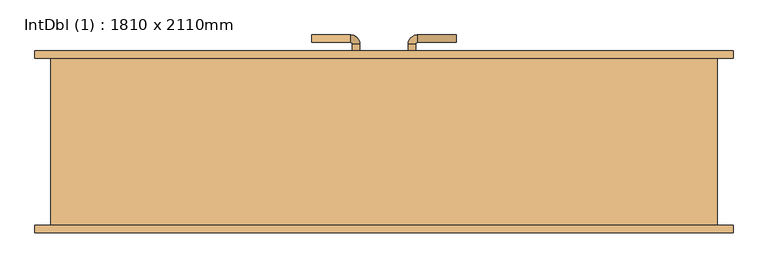
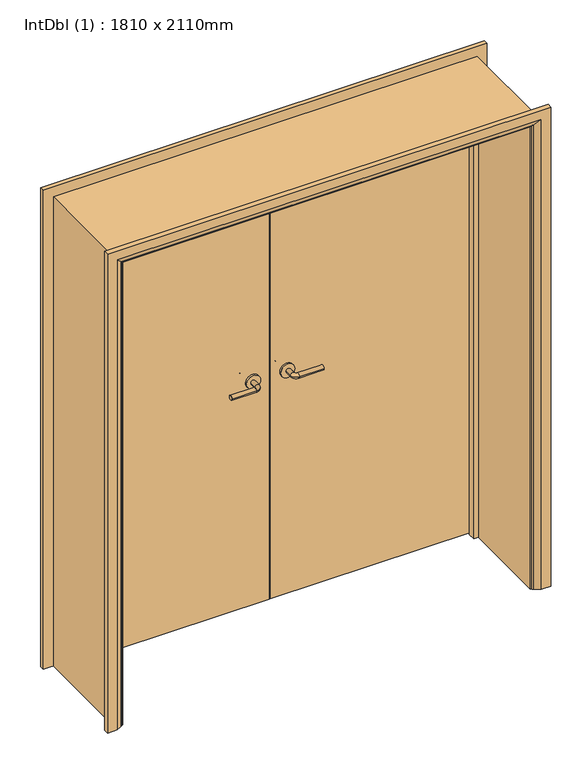
"""IFC4 building model written with IfcOpenShell, lengths in millimetres: door geometry, IntDbl (1) : 1810 x 2110mm."""

from ifc_helpers import new_model, si_unit, point, frame, frame_2d, origin, place, context, project, spatial, polyline, circle_curve, ellipse_curve, trimmed, segment, composite_curve, outline, extrude, faceted_brep, source, transform, mapped, element, save
from ifc_brep_helpers import plane_surface, cylinder_surface, revolved_surface, advanced_brep


def intdbl_1_1810_x_2110mm_24fdf151(model_context):
    return source(origin(), model_context, "Body", "SolidModel", [
        advanced_brep(
        [(-65.0, 185.0, 1007.0), (-85.0, 185.0, 1007.0), (-65.0, 155.0, 1007.0), (-85.0, 155.0, 1007.0), (-90.0, 150.0, 1007.0), (-90.0, 130.0, 1007.0), (-195.0, 130.0, 1007.0), (-195.0, 150.0, 1007.0)],
        [
            (0, 1, circle_curve(frame((-75.0, 185.0, 1007.0), z_axis=(0.0, 1.0, 0.0), x_axis=(-1.0, 0.0, 0.0)), 10.0)),
            (1, 0, circle_curve(frame((-75.0, 185.0, 1007.0), z_axis=(0.0, 1.0, 0.0), x_axis=(-1.0, 0.0, 0.0)), 10.0)),
            (0, 2),
            (2, 3, circle_curve(frame((-75.0, 155.0, 1007.0), z_axis=(0.0, 1.0, 0.0), x_axis=(-1.0, 0.0, 0.0)), 10.0)),
            (3, 1),
            (3, 2, circle_curve(frame((-75.0, 155.0, 1007.0), z_axis=(0.0, 1.0, 0.0), x_axis=(-1.0, 0.0, 0.0)), 10.0)),
            (4, 3, circle_curve(frame((-90.0, 155.0, 1007.0), z_axis=(0.0, 0.0, 1.0), x_axis=(1.0, 0.0, 0.0)), 5.0)),
            (2, 5, circle_curve(frame((-90.0, 155.0, 1007.0), z_axis=(0.0, 0.0, -1.0), x_axis=(1.0, 0.0, 0.0)), 25.0)),
            (5, 4, circle_curve(frame((-90.0, 140.0, 1007.0), z_axis=(1.0, 0.0, 0.0), x_axis=(0.0, 1.0, 0.0)), 10.0)),
            (4, 5, circle_curve(frame((-90.0, 140.0, 1007.0), z_axis=(1.0, 0.0, 0.0), x_axis=(0.0, 1.0, 0.0)), 10.0)),
            (6, 7, circle_curve(frame((-195.0, 140.0, 1007.0), z_axis=(-1.0, 0.0, 0.0), x_axis=(0.0, 1.0, 0.0)), 10.0)),
            (7, 6, circle_curve(frame((-195.0, 140.0, 1007.0), z_axis=(-1.0, 0.0, 0.0), x_axis=(0.0, 1.0, 0.0)), 10.0)),
            (5, 6),
            (7, 4),
        ],
        [
            plane_surface(frame((-75.0, 185.0, 1007.0), z_axis=(0.0, 1.0, 0.0), x_axis=(0.0, 0.0, 1.0))),
            cylinder_surface(frame((-75.0, 185.0, 1007.0), z_axis=(0.0, 1.0, 0.0), x_axis=(-1.0, 0.0, 0.0)), 10.0),
            revolved_surface(trimmed(ellipse_curve(frame((-75.0, 155.0, 1007.0), z_axis=(0.0, 1.0, 0.0), x_axis=(-1.0, 0.0, 0.0)), 10.0, 10.0), [point((-65.0, 155.0, 1007.0))], [point((-85.0, 155.0, 1007.0))], True, "CARTESIAN"), (-90.0, 155.0, 1007.0), (0.0, 0.0, -1.0)),
            revolved_surface(trimmed(ellipse_curve(frame((-75.0, 155.0, 1007.0), z_axis=(0.0, 1.0, 0.0), x_axis=(-1.0, 0.0, 0.0)), 10.0, 10.0), [point((-85.0, 155.0, 1007.0))], [point((-65.0, 155.0, 1007.0))], True, "CARTESIAN"), (-90.0, 155.0, 1007.0), (0.0, 0.0, -1.0)),
            plane_surface(frame((-195.0, 140.0, 1007.0), z_axis=(-1.0, 0.0, 0.0), x_axis=(0.0, 0.0, 1.0))),
            cylinder_surface(frame((-90.0, 140.0, 1007.0), z_axis=(1.0, 0.0, 0.0), x_axis=(0.0, 1.0, 0.0)), 10.0),
        ],
        [
            (0, [[1, 2]]),
            (1, [[-1, 3, 4, 5]]),
            (1, [[-2, -5, 6, -3]]),
            (2, [[7, -4, 8, 9]]),
            (3, [[-8, -6, -7, 10]]),
            (4, [[11, 12]]),
            (5, [[-9, 13, -12, 14]]),
            (5, [[-10, -14, -11, -13]]),
        ],
    ),
        extrude(outline(composite_curve([segment(trimmed(circle_curve(frame_2d((1007.0, -72.5)), 30.0), [point((1007.0, -42.5))], [point((1007.0, -102.5))], False, "CARTESIAN"), True, "CONTINUOUS"), segment(trimmed(circle_curve(frame_2d((1007.0, -72.5)), 30.0), [point((1007.0, -102.5))], [point((1007.0, -42.5))], False, "CARTESIAN"), True, "CONTINUOUS")], self_intersect=False)), frame((0.0, 185.0, 0.0), z_axis=(0.0, 1.0, 0.0), x_axis=(0.0, 0.0, 1.0)), (0.0, 0.0, 1.0), 8.0),
        advanced_brep(
        [(-65.0, 233.0, 1007.0), (-85.0, 233.0, 1007.0), (-85.0, 263.0, 1007.0), (-65.0, 263.0, 1007.0), (-90.0, 268.0, 1007.0), (-90.0, 288.0, 1007.0), (-195.0, 288.0, 1007.0), (-195.0, 268.0, 1007.0)],
        [
            (0, 1, circle_curve(frame((-75.0, 233.0, 1007.0), z_axis=(0.0, -1.0, 0.0), x_axis=(-1.0, 0.0, 0.0)), 10.0)),
            (1, 0, circle_curve(frame((-75.0, 233.0, 1007.0), z_axis=(0.0, -1.0, 0.0), x_axis=(-1.0, 0.0, 0.0)), 10.0)),
            (1, 2),
            (2, 3, circle_curve(frame((-75.0, 263.0, 1007.0), z_axis=(0.0, -1.0, 0.0), x_axis=(-1.0, 0.0, 0.0)), 10.0)),
            (3, 0),
            (3, 2, circle_curve(frame((-75.0, 263.0, 1007.0), z_axis=(0.0, -1.0, 0.0), x_axis=(-1.0, 0.0, 0.0)), 10.0)),
            (4, 5, circle_curve(frame((-90.0, 278.0, 1007.0), z_axis=(1.0, 0.0, 0.0), x_axis=(0.0, -1.0, 0.0)), 10.0)),
            (5, 3, circle_curve(frame((-90.0, 263.0, 1007.0), z_axis=(0.0, 0.0, -1.0), x_axis=(1.0, 0.0, 0.0)), 25.0)),
            (2, 4, circle_curve(frame((-90.0, 263.0, 1007.0), z_axis=(0.0, 0.0, 1.0), x_axis=(1.0, 0.0, 0.0)), 5.0)),
            (5, 4, circle_curve(frame((-90.0, 278.0, 1007.0), z_axis=(1.0, 0.0, 0.0), x_axis=(0.0, -1.0, 0.0)), 10.0)),
            (6, 7, circle_curve(frame((-195.0, 278.0, 1007.0), z_axis=(-1.0, 0.0, 0.0), x_axis=(0.0, -1.0, 0.0)), 10.0)),
            (7, 6, circle_curve(frame((-195.0, 278.0, 1007.0), z_axis=(-1.0, 0.0, 0.0), x_axis=(0.0, -1.0, 0.0)), 10.0)),
            (4, 7),
            (6, 5),
        ],
        [
            plane_surface(frame((-75.0, 233.0, 1007.0), z_axis=(0.0, -1.0, 0.0), x_axis=(0.0, 0.0, 1.0))),
            cylinder_surface(frame((-75.0, 233.0, 1007.0), z_axis=(0.0, -1.0, 0.0), x_axis=(-1.0, 0.0, 0.0)), 10.0),
            revolved_surface(trimmed(ellipse_curve(frame((-75.0, 263.0, 1007.0), z_axis=(0.0, 1.0, 0.0), x_axis=(-1.0, 0.0, 0.0)), 10.0, 10.0), [point((-65.0, 263.0, 1007.0))], [point((-85.0, 263.0, 1007.0))], True, "CARTESIAN"), (-90.0, 263.0, 1007.0), (0.0, 0.0, -1.0)),
            revolved_surface(trimmed(ellipse_curve(frame((-75.0, 263.0, 1007.0), z_axis=(0.0, 1.0, 0.0), x_axis=(-1.0, 0.0, 0.0)), 10.0, 10.0), [point((-85.0, 263.0, 1007.0))], [point((-65.0, 263.0, 1007.0))], True, "CARTESIAN"), (-90.0, 263.0, 1007.0), (0.0, 0.0, -1.0)),
            plane_surface(frame((-195.0, 278.0, 1007.0), z_axis=(-1.0, 0.0, 0.0), x_axis=(0.0, 0.0, 1.0))),
            cylinder_surface(frame((-90.0, 278.0, 1007.0), z_axis=(1.0, 0.0, 0.0), x_axis=(0.0, -1.0, 0.0)), 10.0),
        ],
        [
            (0, [[1, 2]]),
            (1, [[3, 4, 5, -2]]),
            (1, [[-5, 6, -3, -1]]),
            (2, [[7, 8, -4, 9]]),
            (3, [[10, -9, -6, -8]]),
            (4, [[11, 12]]),
            (5, [[13, -11, 14, -7]]),
            (5, [[-14, -12, -13, -10]]),
        ],
    ),
        extrude(outline(composite_curve([segment(trimmed(circle_curve(frame_2d((1007.0, -72.5)), 30.0), [point((1007.0, -42.5))], [point((1007.0, -102.5))], False, "CARTESIAN"), True, "CONTINUOUS"), segment(trimmed(circle_curve(frame_2d((1007.0, -72.5)), 30.0), [point((1007.0, -102.5))], [point((1007.0, -42.5))], False, "CARTESIAN"), True, "CONTINUOUS")], self_intersect=False)), frame((0.0, 225.0, 0.0), z_axis=(0.0, 1.0, 0.0), x_axis=(0.0, 0.0, 1.0)), (0.0, 0.0, 1.0), 8.0),
        advanced_brep(
        [(65.0, 185.0, 1007.0), (85.0, 185.0, 1007.0), (85.0, 155.0, 1007.0), (65.0, 155.0, 1007.0), (90.0, 150.0, 1007.0), (90.0, 130.0, 1007.0), (195.0, 130.0, 1007.0), (195.0, 150.0, 1007.0)],
        [
            (0, 1, circle_curve(frame((75.0, 185.0, 1007.0), z_axis=(0.0, 1.0, 0.0), x_axis=(1.0, 0.0, 0.0)), 10.0)),
            (1, 0, circle_curve(frame((75.0, 185.0, 1007.0), z_axis=(0.0, 1.0, 0.0), x_axis=(1.0, 0.0, 0.0)), 10.0)),
            (1, 2),
            (2, 3, circle_curve(frame((75.0, 155.0, 1007.0), z_axis=(0.0, 1.0, 0.0), x_axis=(1.0, 0.0, 0.0)), 10.0)),
            (3, 0),
            (3, 2, circle_curve(frame((75.0, 155.0, 1007.0), z_axis=(0.0, 1.0, 0.0), x_axis=(1.0, 0.0, 0.0)), 10.0)),
            (4, 5, circle_curve(frame((90.0, 140.0, 1007.0), z_axis=(-1.0, 0.0, 0.0), x_axis=(0.0, 1.0, 0.0)), 10.0)),
            (5, 3, circle_curve(frame((90.0, 155.0, 1007.0), z_axis=(0.0, 0.0, -1.0), x_axis=(-1.0, 0.0, 0.0)), 25.0)),
            (2, 4, circle_curve(frame((90.0, 155.0, 1007.0), z_axis=(0.0, 0.0, 1.0), x_axis=(-1.0, 0.0, 0.0)), 5.0)),
            (5, 4, circle_curve(frame((90.0, 140.0, 1007.0), z_axis=(-1.0, 0.0, 0.0), x_axis=(0.0, 1.0, 0.0)), 10.0)),
            (6, 7, circle_curve(frame((195.0, 140.0, 1007.0), z_axis=(1.0, 0.0, 0.0), x_axis=(0.0, 1.0, 0.0)), 10.0)),
            (7, 6, circle_curve(frame((195.0, 140.0, 1007.0), z_axis=(1.0, 0.0, 0.0), x_axis=(0.0, 1.0, 0.0)), 10.0)),
            (4, 7),
            (6, 5),
        ],
        [
            plane_surface(frame((75.0, 185.0, 1007.0), z_axis=(0.0, 1.0, 0.0), x_axis=(0.0, 0.0, 1.0))),
            cylinder_surface(frame((75.0, 185.0, 1007.0), z_axis=(0.0, 1.0, 0.0), x_axis=(1.0, 0.0, 0.0)), 10.0),
            revolved_surface(trimmed(ellipse_curve(frame((75.0, 155.0, 1007.0), z_axis=(0.0, -1.0, 0.0), x_axis=(1.0, 0.0, 0.0)), 10.0, 10.0), [point((65.0, 155.0, 1007.0))], [point((85.0, 155.0, 1007.0))], True, "CARTESIAN"), (90.0, 155.0, 1007.0), (0.0, 0.0, -1.0)),
            revolved_surface(trimmed(ellipse_curve(frame((75.0, 155.0, 1007.0), z_axis=(0.0, -1.0, 0.0), x_axis=(1.0, 0.0, 0.0)), 10.0, 10.0), [point((85.0, 155.0, 1007.0))], [point((65.0, 155.0, 1007.0))], True, "CARTESIAN"), (90.0, 155.0, 1007.0), (0.0, 0.0, -1.0)),
            plane_surface(frame((195.0, 140.0, 1007.0), z_axis=(1.0, 0.0, 0.0), x_axis=(0.0, 0.0, 1.0))),
            cylinder_surface(frame((90.0, 140.0, 1007.0), z_axis=(-1.0, 0.0, 0.0), x_axis=(0.0, 1.0, 0.0)), 10.0),
        ],
        [
            (0, [[1, 2]]),
            (1, [[3, 4, 5, -2]]),
            (1, [[-5, 6, -3, -1]]),
            (2, [[7, 8, -4, 9]]),
            (3, [[10, -9, -6, -8]]),
            (4, [[11, 12]]),
            (5, [[13, -11, 14, -7]]),
            (5, [[-14, -12, -13, -10]]),
        ],
    ),
        extrude(outline(composite_curve([segment(trimmed(circle_curve(frame_2d((1007.0, 72.5)), 30.0), [point((1007.0, 42.5))], [point((1007.0, 102.5))], False, "CARTESIAN"), True, "CONTINUOUS"), segment(trimmed(circle_curve(frame_2d((1007.0, 72.5)), 30.0), [point((1007.0, 102.5))], [point((1007.0, 42.5))], False, "CARTESIAN"), True, "CONTINUOUS")], self_intersect=False)), frame((0.0, 185.0, 0.0), z_axis=(0.0, 1.0, 0.0), x_axis=(0.0, 0.0, 1.0)), (0.0, 0.0, 1.0), 8.0),
        advanced_brep(
        [(65.0, 233.0, 1007.0), (85.0, 233.0, 1007.0), (65.0, 263.0, 1007.0), (85.0, 263.0, 1007.0), (90.0, 268.0, 1007.0), (90.0, 288.0, 1007.0), (195.0, 288.0, 1007.0), (195.0, 268.0, 1007.0)],
        [
            (0, 1, circle_curve(frame((75.0, 233.0, 1007.0), z_axis=(0.0, -1.0, 0.0), x_axis=(1.0, 0.0, 0.0)), 10.0)),
            (1, 0, circle_curve(frame((75.0, 233.0, 1007.0), z_axis=(0.0, -1.0, 0.0), x_axis=(1.0, 0.0, 0.0)), 10.0)),
            (0, 2),
            (2, 3, circle_curve(frame((75.0, 263.0, 1007.0), z_axis=(0.0, -1.0, 0.0), x_axis=(1.0, 0.0, 0.0)), 10.0)),
            (3, 1),
            (3, 2, circle_curve(frame((75.0, 263.0, 1007.0), z_axis=(0.0, -1.0, 0.0), x_axis=(1.0, 0.0, 0.0)), 10.0)),
            (4, 3, circle_curve(frame((90.0, 263.0, 1007.0), z_axis=(0.0, 0.0, 1.0), x_axis=(-1.0, 0.0, 0.0)), 5.0)),
            (2, 5, circle_curve(frame((90.0, 263.0, 1007.0), z_axis=(0.0, 0.0, -1.0), x_axis=(-1.0, 0.0, 0.0)), 25.0)),
            (5, 4, circle_curve(frame((90.0, 278.0, 1007.0), z_axis=(-1.0, 0.0, 0.0), x_axis=(0.0, -1.0, 0.0)), 10.0)),
            (4, 5, circle_curve(frame((90.0, 278.0, 1007.0), z_axis=(-1.0, 0.0, 0.0), x_axis=(0.0, -1.0, 0.0)), 10.0)),
            (6, 7, circle_curve(frame((195.0, 278.0, 1007.0), z_axis=(1.0, 0.0, 0.0), x_axis=(0.0, -1.0, 0.0)), 10.0)),
            (7, 6, circle_curve(frame((195.0, 278.0, 1007.0), z_axis=(1.0, 0.0, 0.0), x_axis=(0.0, -1.0, 0.0)), 10.0)),
            (5, 6),
            (7, 4),
        ],
        [
            plane_surface(frame((75.0, 233.0, 1007.0), z_axis=(0.0, -1.0, 0.0), x_axis=(0.0, 0.0, 1.0))),
            cylinder_surface(frame((75.0, 233.0, 1007.0), z_axis=(0.0, -1.0, 0.0), x_axis=(1.0, 0.0, 0.0)), 10.0),
            revolved_surface(trimmed(ellipse_curve(frame((75.0, 263.0, 1007.0), z_axis=(0.0, -1.0, 0.0), x_axis=(1.0, 0.0, 0.0)), 10.0, 10.0), [point((65.0, 263.0, 1007.0))], [point((85.0, 263.0, 1007.0))], True, "CARTESIAN"), (90.0, 263.0, 1007.0), (0.0, 0.0, -1.0)),
            revolved_surface(trimmed(ellipse_curve(frame((75.0, 263.0, 1007.0), z_axis=(0.0, -1.0, 0.0), x_axis=(1.0, 0.0, 0.0)), 10.0, 10.0), [point((85.0, 263.0, 1007.0))], [point((65.0, 263.0, 1007.0))], True, "CARTESIAN"), (90.0, 263.0, 1007.0), (0.0, 0.0, -1.0)),
            plane_surface(frame((195.0, 278.0, 1007.0), z_axis=(1.0, 0.0, 0.0), x_axis=(0.0, 0.0, 1.0))),
            cylinder_surface(frame((90.0, 278.0, 1007.0), z_axis=(-1.0, 0.0, 0.0), x_axis=(0.0, -1.0, 0.0)), 10.0),
        ],
        [
            (0, [[1, 2]]),
            (1, [[-1, 3, 4, 5]]),
            (1, [[-2, -5, 6, -3]]),
            (2, [[7, -4, 8, 9]]),
            (3, [[-8, -6, -7, 10]]),
            (4, [[11, 12]]),
            (5, [[-9, 13, -12, 14]]),
            (5, [[-10, -14, -11, -13]]),
        ],
    ),
        extrude(outline(composite_curve([segment(trimmed(circle_curve(frame_2d((1007.0, 72.5)), 30.0), [point((1007.0, 42.5))], [point((1007.0, 102.5))], False, "CARTESIAN"), True, "CONTINUOUS"), segment(trimmed(circle_curve(frame_2d((1007.0, 72.5)), 30.0), [point((1007.0, 102.5))], [point((1007.0, 42.5))], False, "CARTESIAN"), True, "CONTINUOUS")], self_intersect=False)), frame((0.0, 225.0, 0.0), z_axis=(0.0, 1.0, 0.0), x_axis=(0.0, 0.0, 1.0)), (0.0, 0.0, 1.0), 8.0),
        advanced_brep(
        [(-940.0, -245.0, 0.0), (-940.0, -225.0, 0.0), (-870.0, -225.0, 0.0), (-874.0, -231.0, 0.0), (-900.0, -245.0, 0.0), (-940.0, -245.0, 2145.0), (-940.0, -225.0, 2145.0), (940.0, -225.0, 2145.0), (940.0, -225.0, 0.0), (870.0, -225.0, 0.0), (870.0, -225.0, 2075.0), (-870.0, -225.0, 2075.0), (-874.0, -231.0, 2079.0), (-900.0, -245.0, 2105.0), (900.0, -245.0, 2105.0), (900.0, -245.0, 0.0), (940.0, -245.0, 0.0), (940.0, -245.0, 2145.0), (874.0, -231.0, 0.0), (874.0, -231.0, 2079.0)],
        [
            (0, 1),
            (1, 2),
            (2, 3, circle_curve(frame((-878.0, -224.0, 0.0), z_axis=(0.0, 0.0, -1.0), x_axis=(-1.0, 0.0, 0.0)), 8.0622577)),
            (3, 4),
            (4, 0),
            (0, 5),
            (5, 6),
            (6, 1),
            (6, 7),
            (7, 8),
            (8, 9),
            (9, 10),
            (10, 11),
            (11, 2),
            (11, 12, ellipse_curve(frame((-878.0, -224.0, 2083.0), z_axis=(-0.7071067811865475, 0.0, -0.7071067811865475), x_axis=(0.7071067811865474, 0.0, -0.7071067811865476)), 11.4017543, 8.0622577)),
            (12, 3),
            (12, 13),
            (13, 4),
            (13, 14),
            (14, 15),
            (15, 16),
            (16, 17),
            (17, 5),
            (7, 17),
            (16, 8),
            (15, 18),
            (18, 9, circle_curve(frame((878.0, -224.0, 0.0), z_axis=(0.0, 0.0, -1.0), x_axis=(1.0, 0.0, 0.0)), 8.0622577)),
            (19, 10, ellipse_curve(frame((878.0, -224.0, 2083.0), z_axis=(0.7071067811865475, 0.0, -0.7071067811865475), x_axis=(0.7071067811865474, 0.0, 0.7071067811865476)), 11.4017543, 8.0622577)),
            (18, 19),
            (14, 19),
            (19, 12),
        ],
        [
            plane_surface(frame((-870.0, -225.0, 0.0), z_axis=(0.0, 0.0, -1.0), x_axis=(0.0, -1.0, 0.0))),
            plane_surface(frame((-940.0, -245.0, 0.0), z_axis=(-1.0, 0.0, 0.0), x_axis=(0.0, 0.0, 1.0))),
            plane_surface(frame((-940.0, -225.0, 0.0), z_axis=(0.0, 1.0, 0.0), x_axis=(0.0, 0.0, 1.0))),
            cylinder_surface(frame((-878.0, -224.0, 0.0), z_axis=(0.0, 0.0, -1.0), x_axis=(-1.0, 0.0, 0.0)), 8.0622577),
            plane_surface(frame((-874.0, -231.0, 0.0), z_axis=(0.4740998230350183, -0.8804710999221749, 0.0), x_axis=(0.0, 0.0, 1.0))),
            plane_surface(frame((-900.0, -245.0, 0.0), z_axis=(0.0, -1.0, 0.0), x_axis=(0.0, 0.0, 1.0))),
            plane_surface(frame((940.0, -245.0, 2145.0), z_axis=(1.0, 0.0, 0.0), x_axis=(0.0, 0.0, -1.0))),
            plane_surface(frame((870.0, -225.0, 0.0), z_axis=(0.0, 0.0, -1.0), x_axis=(0.0, -1.0, 0.0))),
            cylinder_surface(frame((878.0, -224.0, 2075.0), z_axis=(0.0, 0.0, 1.0), x_axis=(1.0, 0.0, 0.0)), 8.0622577),
            plane_surface(frame((874.0, -231.0, 2079.0), z_axis=(-0.4740998230350183, -0.8804710999221749, 0.0), x_axis=(0.0, 0.0, -1.0))),
            plane_surface(frame((-940.0, -245.0, 2145.0), z_axis=(0.0, 0.0, 1.0), x_axis=(1.0, 0.0, 0.0))),
            cylinder_surface(frame((-870.0, -224.0, 2083.0), z_axis=(-1.0, 0.0, 0.0), x_axis=(0.0, 0.0, 1.0)), 8.0622577),
            plane_surface(frame((-874.0, -231.0, 2079.0), z_axis=(0.0, -0.8804710999221749, -0.4740998230350183), x_axis=(1.0, 0.0, 0.0))),
        ],
        [
            (0, [[1, 2, 3, 4, 5]]),
            (1, [[-1, 6, 7, 8]]),
            (2, [[-2, -8, 9, 10, 11, 12, 13, 14]]),
            (3, [[-3, -14, 15, 16]]),
            (4, [[-4, -16, 17, 18]]),
            (5, [[-5, -18, 19, 20, 21, 22, 23, -6]]),
            (6, [[24, -22, 25, -10]]),
            (7, [[-21, 26, 27, -11, -25]]),
            (8, [[28, -12, -27, 29]]),
            (9, [[30, -29, -26, -20]]),
            (10, [[-7, -23, -24, -9]]),
            (11, [[-15, -13, -28, 31]]),
            (12, [[-17, -31, -30, -19]]),
        ],
    ),
        advanced_brep(
        [(940.0, 245.0, 0.0), (940.0, 225.0, 0.0), (870.0, 225.0, 0.0), (874.0, 231.0, 0.0), (900.0, 245.0, 0.0), (940.0, 245.0, 2145.0), (940.0, 225.0, 2145.0), (-940.0, 225.0, 2145.0), (-940.0, 225.0, 0.0), (-870.0, 225.0, 0.0), (-870.0, 225.0, 2075.0), (870.0, 225.0, 2075.0), (874.0, 231.0, 2079.0), (900.0, 245.0, 2105.0), (-900.0, 245.0, 2105.0), (-900.0, 245.0, 0.0), (-940.0, 245.0, 0.0), (-940.0, 245.0, 2145.0), (-874.0, 231.0, 0.0), (-874.0, 231.0, 2079.0)],
        [
            (0, 1),
            (1, 2),
            (2, 3, circle_curve(frame((878.0, 224.0, 0.0), z_axis=(0.0, 0.0, -1.0), x_axis=(1.0, 0.0, 0.0)), 8.0622577)),
            (3, 4),
            (4, 0),
            (0, 5),
            (5, 6),
            (6, 1),
            (6, 7),
            (7, 8),
            (8, 9),
            (9, 10),
            (10, 11),
            (11, 2),
            (11, 12, ellipse_curve(frame((878.0, 224.0, 2083.0), z_axis=(0.7071067811865475, 0.0, -0.7071067811865475), x_axis=(-0.7071067811865474, 0.0, -0.7071067811865476)), 11.4017543, 8.0622577)),
            (12, 3),
            (12, 13),
            (13, 4),
            (13, 14),
            (14, 15),
            (15, 16),
            (16, 17),
            (17, 5),
            (7, 17),
            (16, 8),
            (15, 18),
            (18, 9, circle_curve(frame((-878.0, 224.0, 0.0), z_axis=(0.0, 0.0, -1.0), x_axis=(-1.0, 0.0, 0.0)), 8.0622577)),
            (19, 10, ellipse_curve(frame((-878.0, 224.0, 2083.0), z_axis=(-0.7071067811865475, 0.0, -0.7071067811865475), x_axis=(-0.7071067811865474, 0.0, 0.7071067811865476)), 11.4017543, 8.0622577)),
            (18, 19),
            (14, 19),
            (19, 12),
        ],
        [
            plane_surface(frame((870.0, 225.0, 0.0), z_axis=(0.0, 0.0, -1.0), x_axis=(0.0, -1.0, 0.0))),
            plane_surface(frame((940.0, 245.0, 0.0), z_axis=(1.0, 0.0, 0.0), x_axis=(0.0, 0.0, 1.0))),
            plane_surface(frame((940.0, 225.0, 0.0), z_axis=(0.0, -1.0, 0.0), x_axis=(0.0, 0.0, 1.0))),
            cylinder_surface(frame((878.0, 224.0, 0.0), z_axis=(0.0, 0.0, -1.0), x_axis=(1.0, 0.0, 0.0)), 8.0622577),
            plane_surface(frame((874.0, 231.0, 0.0), z_axis=(-0.4740998230350126, 0.8804710999221779, 0.0), x_axis=(0.0, 0.0, 1.0))),
            plane_surface(frame((900.0, 245.0, 0.0), z_axis=(0.0, 1.0, 0.0), x_axis=(0.0, 0.0, 1.0))),
            plane_surface(frame((-940.0, 245.0, 2145.0), z_axis=(-1.0, 0.0, 0.0), x_axis=(0.0, 0.0, -1.0))),
            plane_surface(frame((-870.0, 225.0, 0.0), z_axis=(0.0, 0.0, -1.0), x_axis=(0.0, -1.0, 0.0))),
            cylinder_surface(frame((-878.0, 224.0, 2075.0), z_axis=(0.0, 0.0, 1.0), x_axis=(-1.0, 0.0, 0.0)), 8.0622577),
            plane_surface(frame((-874.0, 231.0, 2079.0), z_axis=(0.4740998230350183, 0.8804710999221749, 0.0), x_axis=(0.0, 0.0, -1.0))),
            plane_surface(frame((940.0, 245.0, 2145.0), z_axis=(0.0, 0.0, 1.0), x_axis=(-1.0, 0.0, 0.0))),
            cylinder_surface(frame((870.0, 224.0, 2083.0), z_axis=(1.0, 0.0, 0.0), x_axis=(0.0, 0.0, 1.0)), 8.0622577),
            plane_surface(frame((874.0, 231.0, 2079.0), z_axis=(0.0, 0.8804710999221763, -0.4740998230350154), x_axis=(-1.0, 0.0, 0.0))),
        ],
        [
            (0, [[1, 2, 3, 4, 5]]),
            (1, [[-1, 6, 7, 8]]),
            (2, [[-2, -8, 9, 10, 11, 12, 13, 14]]),
            (3, [[-3, -14, 15, 16]]),
            (4, [[-4, -16, 17, 18]]),
            (5, [[-5, -18, 19, 20, 21, 22, 23, -6]]),
            (6, [[24, -22, 25, -10]]),
            (7, [[-21, 26, 27, -11, -25]]),
            (8, [[28, -12, -27, 29]]),
            (9, [[30, -29, -26, -20]]),
            (10, [[-7, -23, -24, -9]]),
            (11, [[-15, -13, -28, 31]]),
            (12, [[-17, -31, -30, -19]]),
        ],
    ),
        faceted_brep([(-846.0, 190.0, 0.0), (-846.0, 158.0, 0.0), (-865.0, 158.0, 0.0), (-865.0, 190.0, 0.0), (-846.0, 190.0, 2051.0), (-846.0, 158.0, 2051.0), (-865.0, 158.0, 2070.0), (-865.0, 190.0, 2070.0), (846.0, 190.0, 0.0), (865.0, 190.0, 0.0), (865.0, 158.0, 0.0), (846.0, 158.0, 0.0), (846.0, 190.0, 2051.0), (865.0, 190.0, 2070.0), (865.0, 158.0, 2070.0), (846.0, 158.0, 2051.0)], [[[0, 1, 2, 3]], [[1, 0, 4, 5]], [[2, 1, 5, 6]], [[3, 2, 6, 7]], [[0, 3, 7, 4]], [[8, 9, 10, 11]], [[12, 13, 9, 8]], [[13, 14, 10, 9]], [[14, 15, 11, 10]], [[15, 12, 8, 11]], [[5, 4, 12, 15]], [[6, 5, 15, 14]], [[7, 6, 14, 13]], [[4, 7, 13, 12]]]),
        extrude(outline(polyline([(2102.0, -897.0), (0.0, -897.0), (0.0, -865.0), (2070.0, -865.0), (2070.0, 865.0), (0.0, 865.0), (0.0, 897.0), (2102.0, 897.0), (2102.0, -897.0)])), frame((0.0, -225.0, 0.0), z_axis=(0.0, 1.0, 0.0), x_axis=(0.0, 0.0, 1.0)), (0.0, 0.0, 1.0), 450.0),
        extrude(outline(polyline([(-1.5, 193.0), (-862.0, 193.0), (-862.0, 225.0), (-1.5, 225.0), (-1.5, 193.0)])), frame((0.0, 0.0, 5.753223), z_axis=(0.0, 0.0, 1.0), x_axis=(1.0, 0.0, 0.0)), (0.0, 0.0, 1.0), 2061.246777),
        extrude(outline(polyline([(862.0, 193.0), (1.5, 193.0), (1.5, 225.0), (862.0, 225.0), (862.0, 193.0)])), frame((0.0, 0.0, 5.753223), z_axis=(0.0, 0.0, 1.0), x_axis=(1.0, 0.0, 0.0)), (0.0, 0.0, 1.0), 2061.246777),
    ])


if __name__ == "__main__":
    model = new_model("IFC4")
    model_context = context("Model", 3, world=origin())
    ifc_project = project(units=[si_unit("LENGTHUNIT", "METRE", prefix="MILLI")], contexts=[model_context])
    site = spatial("IfcSite", under=ifc_project)
    building = spatial("IfcBuilding", under=site)
    placement = place(None, origin())
    intdbl_1_1810_x_2110mm_shape = intdbl_1_1810_x_2110mm_24fdf151(model_context)
    element("IfcDoor", 1, ObjectType="IntDbl (1) : 1810 x 2110mm", at=placement, inside=building, context=model_context, shape_type="MappedRepresentation", body=[
        mapped(intdbl_1_1810_x_2110mm_shape, transform((0.0, 0.0, 0.0), x_axis=(1.0, 0.0, 0.0), y_axis=(0.0, 1.0, 0.0), z_axis=(0.0, 0.0, 1.0))),
    ])
    save(model, "model.ifc")

# Revit data of these elements
# Type "IntDbl (1) : 1810 x 2110mm"
#   Type Mark = "34"
#   Type Comments = "Internal Double"
#   Operation = "DoubleDoorSingleSwing"
#   Keynote = "L20"
#   Description = "Internal Double Door"
#   Thickness = 32 mm
#   Stop Thickness = 19 mm
#   Stop Depth = 32 mm
#   Rough Width = 1810 mm
#   Rough Height = 2110 mm
#   Handle Z Distance = 1000 mm
#   Handle X Distance = 75 mm
#   Frame Thickness = 32 mm
#   Door Panel Width = 860.5 mm
#   Door Panel Thickness = 32 mm
#   Door Panel Height = 2060 mm
#   Height = 2110 mm
#   Door Panel Offset = 0 mm
#   Structural Tolerance = 8 mm
#   Tolerance = 3 mm
#   UnderCut = 7 mm
#   Width = 1810 mm
#   Architrave Setback = 5 mm
#   Vis - Ironmongery = yes
#   Material Ironmongery = Door - Handle
#   Material Glass = Door - Glazing
#   Material Frame = Door - Frame/Mullion
#   Material Door = Door - Panel
#   Material Architrave = Door - Architrave
#   Function = (empty or 0)
#   Wall Closure = (empty or 0)
# Element 1 (IfcDoor, "IntDbl (1) : 1810 x 2110mm")
#   Materials on its faces: "Door - Handle", "Door - Architrave", "Door - Frame/Mullion", "Door - Panel"
# Materials
#   "Door - Handle": class "Miscellaneous", colour RGB 0 0 0, transparency 0
#   "Door - Glazing": class "Miscellaneous", colour RGB 0 0 255, transparency 0.75
#   "Door - Frame/Mullion": class "Wood", colour RGB 212 179 113, transparency 0
#   "Door - Panel": class "Wood", colour RGB 210 159 95, transparency 0
#   "Door - Architrave": class "Wood", colour RGB 154 90 5, transparency 0
